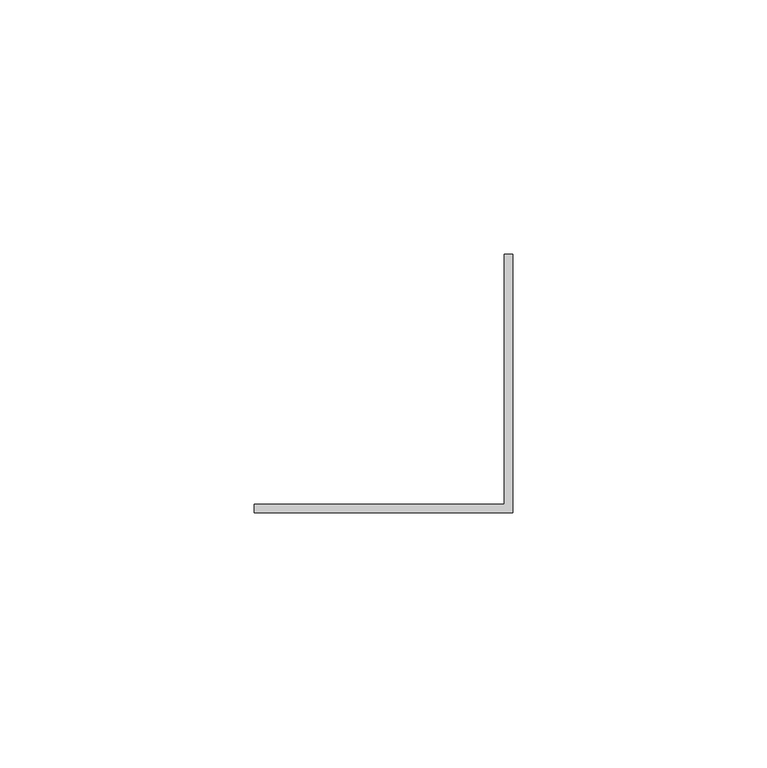
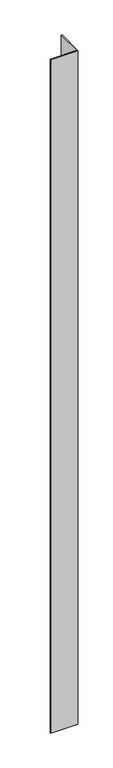
"""IFC4 building model written with IfcOpenShell, lengths in millimetres: proxy geometry, Generic Models 2:Generic Models 2:310765:Generic Models 2:310765 : Generic Models 2:Generic Models 2:310765:58 : Generic Models 2:Generic Models 2:310765:Generic Models 2:310765 : Generic Models 2:Generic Models 2:310765:300385."""

from ifc_helpers import new_model, si_unit, frame, origin, place, context, project, spatial, polyline, outline, extrude, source, transform, mapped, element, save


def generic_models_e0eb15f6(model_context):
    return source(origin(), model_context, "Body", "SweptSolid", [
        extrude(outline(polyline([(579067.3390043, -578760.1501539), (579016.5390043, -578760.1501539), (579016.5390043, -578758.5626539), (579065.7515043, -578758.5626539), (579065.7515043, -578709.3501539), (579067.3390043, -578709.3501539), (579067.3390043, -578760.1501539)])), frame((0.0, 0.0, 4828.849258), z_axis=(0.0, 0.0, 1.0), x_axis=(1.0, 0.0, 0.0)), (0.0, 0.0, 1.0), 1324.3203982),
    ])


if __name__ == "__main__":
    model = new_model("IFC4")
    model_context = context("Model", 3, world=origin())
    ifc_project = project(units=[si_unit("LENGTHUNIT", "METRE", prefix="MILLI")], contexts=[model_context])
    site = spatial("IfcSite", under=ifc_project)
    building = spatial("IfcBuilding", under=site)
    placement = place(None, origin())
    generic_models_shape = generic_models_e0eb15f6(model_context)
    element("IfcBuildingElementProxy", 1, Name="Generic Models 2:Generic Models 2:310765:Generic Models 2:310765 : Generic Models 2:Generic Models 2:310765:58 : Generic Models 2:Generic Models 2:310765:Generic Models 2:310765 : Generic Models 2:Generic Models 2:310765:300385", ObjectType="Generic Models 2:Generic Models 2:310765:Generic Models 2:310765 : Generic Models 2:Generic Models 2:310765:58 : Generic Models 2:Generic Models 2:310765:Generic Models 2:310765 : Generic Models 2:Generic Models 2:310765:300385", at=placement, inside=building, context=model_context, shape_type="MappedRepresentation", body=[
        mapped(generic_models_shape, transform((0.0, 0.0, 0.0), x_axis=(1.0, 0.0, 0.0), y_axis=(0.0, 1.0, 0.0), z_axis=(0.0, 0.0, 1.0))),
    ])
    save(model, "model.ifc")

# Revit data of these elements
# Type "Generic Models 2:Generic Models 2:310765:Generic Models 2:310765 : Generic Models 2:Generic Models 2:310765:58 : Generic Models 2:Generic Models 2:310765:Generic Models 2:310765 : Generic Models 2:Generic Models 2:310765:300385"
#   NameOverride = "Generic Models 2:Generic Models 2:310765:Generic Models 2:310765 : Generic Models 2:Generic Models 2:310765:300385"
#   ObjectTypeOverride = "Generic Models 2:310765 : Generic Models 2:Generic Models 2:310765"
#   Reference = "Generic Models 2"
#   Tag = "300385"
# Element 1 (IfcBuildingElementProxy, "Generic Models 2:Generic Models 2:310765:Generic Models 2:310765 : Generic Models 2:Generic Models 2:310765:58 : Generic Models 2:Generic Models 2:310765:Generic Models 2:310765 : Generic Models 2:Generic Models 2:310765:300385")
#   Materials on its faces: "BRAKE METAL CLOSURE TRIM"
# Materials
#   "BRAKE METAL CLOSURE TRIM": class "Unassigned", colour RGB 182 182 182, transparency 0, Cost = 0
